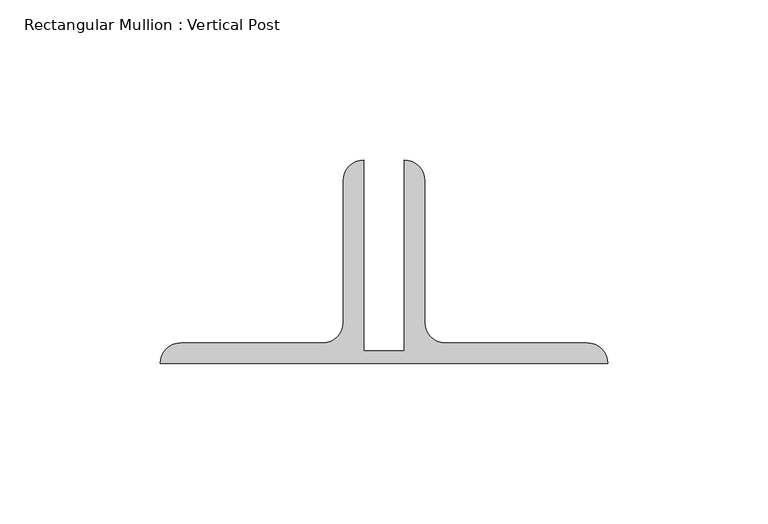
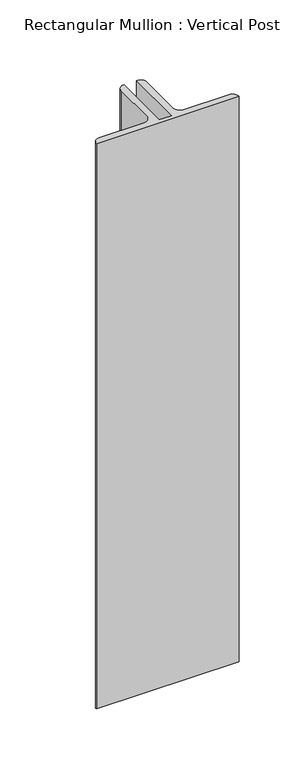
"""IFC4 building model written with IfcOpenShell, lengths in millimetres: member geometry, Rectangular Mullion : Vertical Post."""

import ifcopenshell
import ifcopenshell.guid

model = None  # the IFC model being written
_history = None  # IfcOwnerHistory: only IFC2X3 demands one
_inside = {}  # id of a spatial element -> (the spatial element, [elements in it])
_under = {}  # id of a project, library or spatial element -> (it, [spatial elements below it])
_declared = {}  # id of a project -> (the project, [libraries it declares])
_typed = {}  # id of a type object -> (the type object, [elements of that type])
_made_of = {}  # id of a material, layer set ... -> (it, [elements and type objects made of it])


def new_model(schema):
    """Start an empty IFC model of exactly this schema.

    Asked for "IFC4X3", IfcOpenShell would pick the latest addendum, in which some entities
    have other attributes; the version numbers below select the first issue.
    IFC2X3 requires an IfcOwnerHistory on every rooted entity: one is made here for all.
    """
    global model, _history
    if schema == "IFC4X3":
        model = ifcopenshell.file(schema_version=(4, 3, 0, 0))
    else:
        model = ifcopenshell.file(schema=schema)
    _inside.clear()
    _under.clear()
    _declared.clear()
    _typed.clear()
    _made_of.clear()
    _history = None
    if model.schema == "IFC2X3":
        org = make("IfcOrganization", Name="unknown")
        user = make(
            "IfcPersonAndOrganization",
            ThePerson=make("IfcPerson", FamilyName="unknown"),
            TheOrganization=org,
        )
        app = make(
            "IfcApplication",
            ApplicationDeveloper=org,
            Version="unknown",
            ApplicationFullName="unknown",
            ApplicationIdentifier="unknown",
        )
        _history = make(
            "IfcOwnerHistory",
            OwningUser=user,
            OwningApplication=app,
            ChangeAction="ADDED",
            CreationDate=0,
        )
    return model


def make(cls, **values):
    """One entity of the class cls with the attributes given. An attribute that is None is left unset."""
    return model.create_entity(
        cls, **{name: value for name, value in values.items() if value is not None}
    )


def rooted(cls, **values):
    """An entity with a GlobalId (a new one), such as an element, a storey or a relation."""
    return make(cls, GlobalId=ifcopenshell.guid.new(), OwnerHistory=_history, **values)


def si_unit(unit_type, name, prefix=None):
    """IfcSIUnit, for example si_unit("LENGTHUNIT", "METRE", prefix="MILLI")."""
    return make("IfcSIUnit", UnitType=unit_type, Prefix=prefix, Name=name)


def assignment(units):
    """IfcUnitAssignment: the units of a project."""
    return None if units is None else make("IfcUnitAssignment", Units=units)


def point(xyz):
    """IfcCartesianPoint."""
    return None if xyz is None else make("IfcCartesianPoint", Coordinates=xyz)


def direction(xyz):
    """IfcDirection."""
    return None if xyz is None else make("IfcDirection", DirectionRatios=xyz)


def frame(location, z_axis=None, x_axis=None):
    """IfcAxis2Placement3D, a coordinate frame: its origin and axes. An axis left out is left unset."""
    return make(
        "IfcAxis2Placement3D",
        Location=point(location),
        Axis=direction(z_axis),
        RefDirection=direction(x_axis),
    )


def frame_2d(location, x_axis=None):
    """IfcAxis2Placement2D, a coordinate frame in the plane: its origin and x axis."""
    return make(
        "IfcAxis2Placement2D", Location=point(location), RefDirection=direction(x_axis)
    )


def origin():
    """The frame at (0, 0, 0) with its axes left unset."""
    return frame((0.0, 0.0, 0.0))


def place(relative_to, where):
    """IfcLocalPlacement: puts the frame where relative to a parent placement (None: the world)."""
    return make(
        "IfcLocalPlacement", PlacementRelTo=relative_to, RelativePlacement=where
    )


def context(
    kind, dimensions, precision=None, world=None, true_north=None, identifier=None
):
    """IfcGeometricRepresentationContext, for example the 3D "Model" context."""
    return make(
        "IfcGeometricRepresentationContext",
        ContextIdentifier=identifier,
        ContextType=kind,
        CoordinateSpaceDimension=dimensions,
        Precision=precision,
        WorldCoordinateSystem=world,
        TrueNorth=true_north,
    )


def project(units=None, contexts=None):
    """IfcProject with its units and contexts."""
    return rooted(
        "IfcProject",
        Name="project",
        RepresentationContexts=contexts,
        UnitsInContext=assignment(units),
    )


def spatial(cls, under=None, at=None, **own):
    """A site, building, storey or space (cls), placed at a placement, below another one or the project."""
    s = rooted(cls, ObjectPlacement=at, **own)
    if under is not None:
        _under.setdefault(under.id(), (under, []))[1].append(s)
    return s


def polyline(points):
    """IfcPolyline through the points."""
    return make("IfcPolyline", Points=[point(p) for p in points])


def circle_curve(where, radius):
    """IfcCircle in the frame where."""
    return make("IfcCircle", Position=where, Radius=radius)


def trimmed(basis, trim1, trim2, sense, master):
    """IfcTrimmedCurve: the piece of a basis curve between two trims."""
    return make(
        "IfcTrimmedCurve",
        BasisCurve=basis,
        Trim1=trim1,
        Trim2=trim2,
        SenseAgreement=sense,
        MasterRepresentation=master,
    )


def segment(curve, same_sense, transition):
    """IfcCompositeCurveSegment."""
    return make(
        "IfcCompositeCurveSegment",
        Transition=transition,
        SameSense=same_sense,
        ParentCurve=curve,
    )


def composite_curve(segments, self_intersect=None):
    """IfcCompositeCurve: segments joined end to end."""
    return make("IfcCompositeCurve", Segments=segments, SelfIntersect=self_intersect)


def outline(outer, holes=None, kind="AREA"):
    """IfcArbitraryClosedProfileDef: a profile drawn as a closed curve; with holes, ...WithVoids."""
    if holes is None:
        return make("IfcArbitraryClosedProfileDef", ProfileType=kind, OuterCurve=outer)
    return make(
        "IfcArbitraryProfileDefWithVoids",
        ProfileType=kind,
        OuterCurve=outer,
        InnerCurves=holes,
    )


def extrude(swept, where, along, depth):
    """IfcExtrudedAreaSolid: the profile swept, set in the frame where, extruded along a direction by depth."""
    return make(
        "IfcExtrudedAreaSolid",
        SweptArea=swept,
        Position=where,
        ExtrudedDirection=direction(along),
        Depth=depth,
    )


def shape(context_of_items, identifier, shape_type, items):
    """IfcShapeRepresentation: the items that make up one representation, for example the "Body"."""
    return make(
        "IfcShapeRepresentation",
        ContextOfItems=context_of_items,
        RepresentationIdentifier=identifier,
        RepresentationType=shape_type,
        Items=items,
    )


def source(mapping_origin, context_of_items, identifier, shape_type, items):
    """IfcRepresentationMap: a shape defined once, which mapped items show again and again."""
    return make(
        "IfcRepresentationMap",
        MappingOrigin=mapping_origin,
        MappedRepresentation=shape(context_of_items, identifier, shape_type, items),
    )


def transform(
    local_origin,
    x_axis=None,
    y_axis=None,
    z_axis=None,
    scale=None,
    scale2=None,
    scale3=None,
    uniform=True,
):
    """IfcCartesianTransformationOperator3D, or its non-uniform kind. x_axis, y_axis, z_axis: its Axis1, 2, 3."""
    if uniform:
        return make(
            "IfcCartesianTransformationOperator3D",
            Axis1=direction(x_axis),
            Axis2=direction(y_axis),
            LocalOrigin=point(local_origin),
            Scale=scale,
            Axis3=direction(z_axis),
        )
    return make(
        "IfcCartesianTransformationOperator3DnonUniform",
        Axis1=direction(x_axis),
        Axis2=direction(y_axis),
        LocalOrigin=point(local_origin),
        Scale=scale,
        Axis3=direction(z_axis),
        Scale2=scale2,
        Scale3=scale3,
    )


def mapped(mapping_source, mapping_target):
    """IfcMappedItem: shows the shape of a source again, moved by a transform."""
    return make(
        "IfcMappedItem", MappingSource=mapping_source, MappingTarget=mapping_target
    )


def made_of(thing, what):
    """Note that an element or type object is made of a material, layer set ...; save() writes the relation."""
    if what is not None:
        _made_of.setdefault(what.id(), (what, []))[1].append(thing)
    return thing


def element(
    cls,
    number,
    at=None,
    inside=None,
    cuts=None,
    type_object=None,
    material=None,
    context=None,
    identifier="Body",
    shape_type=None,
    held_by="IfcProductDefinitionShape",
    body=None,
    shapes=None,
    **own,
):
    """One element of the class cls, such as IfcWall. Its Tag is "e" and its number.

    at: its placement. inside: the storey or other place that contains it. cuts: it is an
    opening in that element (IfcRelVoidsElement). A single representation is given by context,
    identifier, shape_type and body (its items); several are given by shapes. held_by: the class
    of the entity that holds the representations. save() writes the other relations.
    """
    e = rooted(cls, Tag="e%d" % number, ObjectPlacement=at, **own)
    if body is not None:
        shapes = [shape(context, identifier, shape_type, body)]
    if shapes is not None:
        e.Representation = make(held_by, Representations=shapes)
    if inside is not None:
        _inside.setdefault(inside.id(), (inside, []))[1].append(e)
    if cuts is not None:
        rooted(
            "IfcRelVoidsElement", RelatingBuildingElement=cuts, RelatedOpeningElement=e
        )
    if type_object is not None:
        _typed.setdefault(type_object.id(), (type_object, []))[1].append(e)
    return made_of(e, material)


def aggregate(whole, parts):
    """IfcRelAggregates: a whole, such as a stair, and the parts it consists of."""
    return rooted("IfcRelAggregates", RelatingObject=whole, RelatedObjects=parts)


def save(model, path):
    """Write the relations noted so far, then the file.

    IfcRelAggregates (storeys below a building ...), IfcRelContainedInSpatialStructure (elements
    in a storey), IfcRelDefinesByType, IfcRelAssociatesMaterial and IfcRelDeclares: one each for
    every whole, place, type object, material and project.
    """
    for whole, parts in _under.values():
        aggregate(whole, parts)
    for where, things in _inside.values():
        rooted(
            "IfcRelContainedInSpatialStructure",
            RelatedElements=things,
            RelatingStructure=where,
        )
    for kind, things in _typed.values():
        rooted("IfcRelDefinesByType", RelatedObjects=things, RelatingType=kind)
    for what, things in _made_of.values():
        rooted("IfcRelAssociatesMaterial", RelatedObjects=things, RelatingMaterial=what)
    for by, libraries in _declared.values():
        rooted("IfcRelDeclares", RelatingContext=by, RelatedDefinitions=libraries)
    model.write(path)


def rectangular_mullion_vertical_post_5424decc(model_context):
    return source(origin(), model_context, "Body", "SweptSolid", [
        extrude(outline(composite_curve([segment(polyline([(-6.35, 22.9145205), (6.35, 22.9145205), (6.35, 82.55)]), True, "CONTINUOUS"), segment(trimmed(circle_curve(frame_2d((6.35, 76.2)), 6.35), [point((6.35, 82.55))], [point((12.7, 76.2))], False, "CARTESIAN"), True, "CONTINUOUS"), segment(polyline([(12.7, 76.2), (12.7, 31.75)]), True, "CONTINUOUS"), segment(trimmed(circle_curve(frame_2d((19.05, 31.75)), 6.35), [point((12.7, 31.75))], [point((19.05, 25.4))], True, "CARTESIAN"), True, "CONTINUOUS"), segment(polyline([(19.05, 25.4), (63.5, 25.4)]), True, "CONTINUOUS"), segment(trimmed(circle_curve(frame_2d((63.5, 19.05)), 6.35), [point((63.5, 25.4))], [point((69.85, 19.05))], False, "CARTESIAN"), True, "CONTINUOUS"), segment(polyline([(69.85, 19.05), (-69.85, 19.05)]), True, "CONTINUOUS"), segment(trimmed(circle_curve(frame_2d((-63.5, 19.05)), 6.35), [point((-69.85, 19.05))], [point((-63.5, 25.4))], False, "CARTESIAN"), True, "CONTINUOUS"), segment(polyline([(-63.5, 25.4), (-19.05, 25.4)]), True, "CONTINUOUS"), segment(trimmed(circle_curve(frame_2d((-19.05, 31.75)), 6.35), [point((-19.05, 25.4))], [point((-12.7, 31.75))], True, "CARTESIAN"), True, "CONTINUOUS"), segment(polyline([(-12.7, 31.75), (-12.7, 76.2)]), True, "CONTINUOUS"), segment(trimmed(circle_curve(frame_2d((-6.35, 76.2)), 6.35), [point((-12.7, 76.2))], [point((-6.35, 82.55))], False, "CARTESIAN"), True, "CONTINUOUS"), segment(polyline([(-6.35, 82.55), (-6.35, 22.9145205)]), True, "CONTINUOUS")], self_intersect=False)), frame((0.0, 0.0, -584.3306001), z_axis=(0.0, 0.0, 1.0), x_axis=(1.0, 0.0, 0.0)), (0.0, 0.0, 1.0), 584.3306001),
    ])


if __name__ == "__main__":
    model = new_model("IFC4")
    model_context = context("Model", 3, world=origin())
    ifc_project = project(units=[si_unit("LENGTHUNIT", "METRE", prefix="MILLI")], contexts=[model_context])
    site = spatial("IfcSite", under=ifc_project)
    building = spatial("IfcBuilding", under=site)
    placement = place(None, origin())
    rectangular_mullion_vertical_post_shape = rectangular_mullion_vertical_post_5424decc(model_context)
    element("IfcMember", 1, ObjectType="Rectangular Mullion : Vertical Post", at=placement, inside=building, context=model_context, shape_type="MappedRepresentation", body=[
        mapped(rectangular_mullion_vertical_post_shape, transform((0.0, 0.0, 0.0), x_axis=(1.0, 0.0, 0.0), y_axis=(0.0, 1.0, 0.0), z_axis=(0.0, 0.0, 1.0))),
    ])
    save(model, "model.ifc")

# Revit data of these elements
# Type "Rectangular Mullion : Vertical Post"
#   built-in parameter 1007351 = -0.0625 (stored number, unit not read)
#   built-in parameter 1007322 = 0.0126789 (stored number, unit not read)
#   built-in parameter 1007321 = 0.229167 (stored number, unit not read)
#   built-in parameter 1007320 = 0.229167 (stored number, unit not read)
# Element 1 (IfcMember, "Rectangular Mullion : Vertical Post")
#   Materials on its faces: "GATE POST: GALVANIZED ANGLES"
# Materials
#   "GATE POST: GALVANIZED ANGLES": class "Unassigned", colour RGB 120 120 120, transparency 0, Cost = 0
